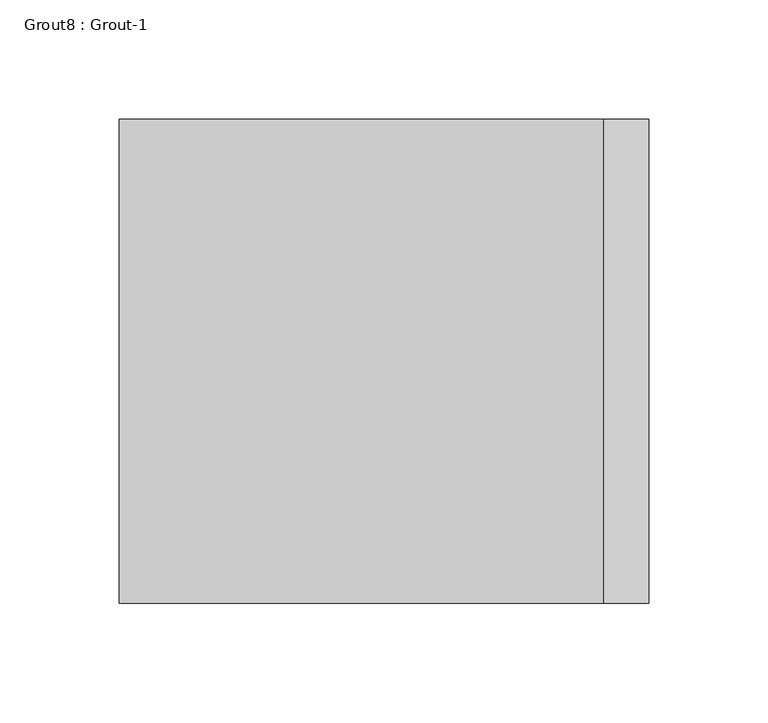
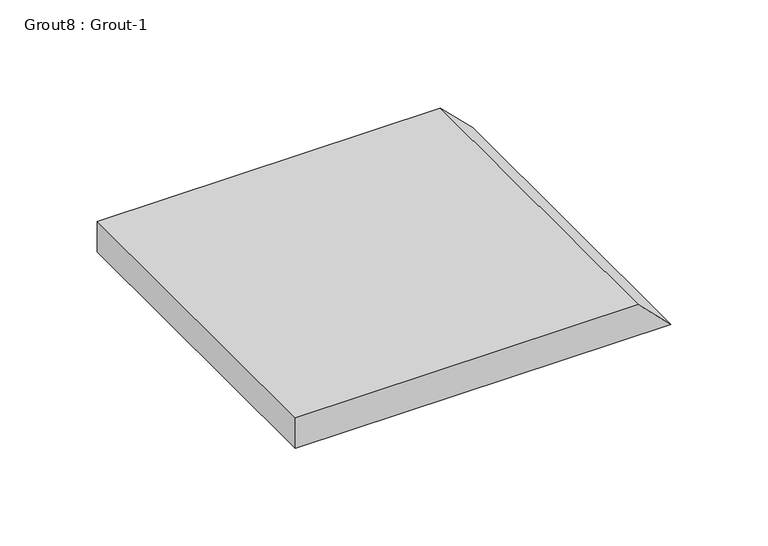
"""IFC4 building model written with IfcOpenShell, lengths in millimetres: proxy geometry, Grout8 : Grout-1."""

import ifcopenshell
import ifcopenshell.guid

model = None  # the IFC model being written
_history = None  # IfcOwnerHistory: only IFC2X3 demands one
_inside = {}  # id of a spatial element -> (the spatial element, [elements in it])
_under = {}  # id of a project, library or spatial element -> (it, [spatial elements below it])
_declared = {}  # id of a project -> (the project, [libraries it declares])
_typed = {}  # id of a type object -> (the type object, [elements of that type])
_made_of = {}  # id of a material, layer set ... -> (it, [elements and type objects made of it])


def new_model(schema):
    """Start an empty IFC model of exactly this schema.

    Asked for "IFC4X3", IfcOpenShell would pick the latest addendum, in which some entities
    have other attributes; the version numbers below select the first issue.
    IFC2X3 requires an IfcOwnerHistory on every rooted entity: one is made here for all.
    """
    global model, _history
    if schema == "IFC4X3":
        model = ifcopenshell.file(schema_version=(4, 3, 0, 0))
    else:
        model = ifcopenshell.file(schema=schema)
    _inside.clear()
    _under.clear()
    _declared.clear()
    _typed.clear()
    _made_of.clear()
    _history = None
    if model.schema == "IFC2X3":
        org = make("IfcOrganization", Name="unknown")
        user = make(
            "IfcPersonAndOrganization",
            ThePerson=make("IfcPerson", FamilyName="unknown"),
            TheOrganization=org,
        )
        app = make(
            "IfcApplication",
            ApplicationDeveloper=org,
            Version="unknown",
            ApplicationFullName="unknown",
            ApplicationIdentifier="unknown",
        )
        _history = make(
            "IfcOwnerHistory",
            OwningUser=user,
            OwningApplication=app,
            ChangeAction="ADDED",
            CreationDate=0,
        )
    return model


def make(cls, **values):
    """One entity of the class cls with the attributes given. An attribute that is None is left unset."""
    return model.create_entity(
        cls, **{name: value for name, value in values.items() if value is not None}
    )


def rooted(cls, **values):
    """An entity with a GlobalId (a new one), such as an element, a storey or a relation."""
    return make(cls, GlobalId=ifcopenshell.guid.new(), OwnerHistory=_history, **values)


def si_unit(unit_type, name, prefix=None):
    """IfcSIUnit, for example si_unit("LENGTHUNIT", "METRE", prefix="MILLI")."""
    return make("IfcSIUnit", UnitType=unit_type, Prefix=prefix, Name=name)


def assignment(units):
    """IfcUnitAssignment: the units of a project."""
    return None if units is None else make("IfcUnitAssignment", Units=units)


def point(xyz):
    """IfcCartesianPoint."""
    return None if xyz is None else make("IfcCartesianPoint", Coordinates=xyz)


def direction(xyz):
    """IfcDirection."""
    return None if xyz is None else make("IfcDirection", DirectionRatios=xyz)


def frame(location, z_axis=None, x_axis=None):
    """IfcAxis2Placement3D, a coordinate frame: its origin and axes. An axis left out is left unset."""
    return make(
        "IfcAxis2Placement3D",
        Location=point(location),
        Axis=direction(z_axis),
        RefDirection=direction(x_axis),
    )


def origin():
    """The frame at (0, 0, 0) with its axes left unset."""
    return frame((0.0, 0.0, 0.0))


def place(relative_to, where):
    """IfcLocalPlacement: puts the frame where relative to a parent placement (None: the world)."""
    return make(
        "IfcLocalPlacement", PlacementRelTo=relative_to, RelativePlacement=where
    )


def context(
    kind, dimensions, precision=None, world=None, true_north=None, identifier=None
):
    """IfcGeometricRepresentationContext, for example the 3D "Model" context."""
    return make(
        "IfcGeometricRepresentationContext",
        ContextIdentifier=identifier,
        ContextType=kind,
        CoordinateSpaceDimension=dimensions,
        Precision=precision,
        WorldCoordinateSystem=world,
        TrueNorth=true_north,
    )


def project(units=None, contexts=None):
    """IfcProject with its units and contexts."""
    return rooted(
        "IfcProject",
        Name="project",
        RepresentationContexts=contexts,
        UnitsInContext=assignment(units),
    )


def spatial(cls, under=None, at=None, **own):
    """A site, building, storey or space (cls), placed at a placement, below another one or the project."""
    s = rooted(cls, ObjectPlacement=at, **own)
    if under is not None:
        _under.setdefault(under.id(), (under, []))[1].append(s)
    return s


def polyline(points):
    """IfcPolyline through the points."""
    return make("IfcPolyline", Points=[point(p) for p in points])


def outline(outer, holes=None, kind="AREA"):
    """IfcArbitraryClosedProfileDef: a profile drawn as a closed curve; with holes, ...WithVoids."""
    if holes is None:
        return make("IfcArbitraryClosedProfileDef", ProfileType=kind, OuterCurve=outer)
    return make(
        "IfcArbitraryProfileDefWithVoids",
        ProfileType=kind,
        OuterCurve=outer,
        InnerCurves=holes,
    )


def extrude(swept, where, along, depth):
    """IfcExtrudedAreaSolid: the profile swept, set in the frame where, extruded along a direction by depth."""
    return make(
        "IfcExtrudedAreaSolid",
        SweptArea=swept,
        Position=where,
        ExtrudedDirection=direction(along),
        Depth=depth,
    )


def shape(context_of_items, identifier, shape_type, items):
    """IfcShapeRepresentation: the items that make up one representation, for example the "Body"."""
    return make(
        "IfcShapeRepresentation",
        ContextOfItems=context_of_items,
        RepresentationIdentifier=identifier,
        RepresentationType=shape_type,
        Items=items,
    )


def source(mapping_origin, context_of_items, identifier, shape_type, items):
    """IfcRepresentationMap: a shape defined once, which mapped items show again and again."""
    return make(
        "IfcRepresentationMap",
        MappingOrigin=mapping_origin,
        MappedRepresentation=shape(context_of_items, identifier, shape_type, items),
    )


def transform(
    local_origin,
    x_axis=None,
    y_axis=None,
    z_axis=None,
    scale=None,
    scale2=None,
    scale3=None,
    uniform=True,
):
    """IfcCartesianTransformationOperator3D, or its non-uniform kind. x_axis, y_axis, z_axis: its Axis1, 2, 3."""
    if uniform:
        return make(
            "IfcCartesianTransformationOperator3D",
            Axis1=direction(x_axis),
            Axis2=direction(y_axis),
            LocalOrigin=point(local_origin),
            Scale=scale,
            Axis3=direction(z_axis),
        )
    return make(
        "IfcCartesianTransformationOperator3DnonUniform",
        Axis1=direction(x_axis),
        Axis2=direction(y_axis),
        LocalOrigin=point(local_origin),
        Scale=scale,
        Axis3=direction(z_axis),
        Scale2=scale2,
        Scale3=scale3,
    )


def mapped(mapping_source, mapping_target):
    """IfcMappedItem: shows the shape of a source again, moved by a transform."""
    return make(
        "IfcMappedItem", MappingSource=mapping_source, MappingTarget=mapping_target
    )


def made_of(thing, what):
    """Note that an element or type object is made of a material, layer set ...; save() writes the relation."""
    if what is not None:
        _made_of.setdefault(what.id(), (what, []))[1].append(thing)
    return thing


def element(
    cls,
    number,
    at=None,
    inside=None,
    cuts=None,
    type_object=None,
    material=None,
    context=None,
    identifier="Body",
    shape_type=None,
    held_by="IfcProductDefinitionShape",
    body=None,
    shapes=None,
    **own,
):
    """One element of the class cls, such as IfcWall. Its Tag is "e" and its number.

    at: its placement. inside: the storey or other place that contains it. cuts: it is an
    opening in that element (IfcRelVoidsElement). A single representation is given by context,
    identifier, shape_type and body (its items); several are given by shapes. held_by: the class
    of the entity that holds the representations. save() writes the other relations.
    """
    e = rooted(cls, Tag="e%d" % number, ObjectPlacement=at, **own)
    if body is not None:
        shapes = [shape(context, identifier, shape_type, body)]
    if shapes is not None:
        e.Representation = make(held_by, Representations=shapes)
    if inside is not None:
        _inside.setdefault(inside.id(), (inside, []))[1].append(e)
    if cuts is not None:
        rooted(
            "IfcRelVoidsElement", RelatingBuildingElement=cuts, RelatedOpeningElement=e
        )
    if type_object is not None:
        _typed.setdefault(type_object.id(), (type_object, []))[1].append(e)
    return made_of(e, material)


def aggregate(whole, parts):
    """IfcRelAggregates: a whole, such as a stair, and the parts it consists of."""
    return rooted("IfcRelAggregates", RelatingObject=whole, RelatedObjects=parts)


def save(model, path):
    """Write the relations noted so far, then the file.

    IfcRelAggregates (storeys below a building ...), IfcRelContainedInSpatialStructure (elements
    in a storey), IfcRelDefinesByType, IfcRelAssociatesMaterial and IfcRelDeclares: one each for
    every whole, place, type object, material and project.
    """
    for whole, parts in _under.values():
        aggregate(whole, parts)
    for where, things in _inside.values():
        rooted(
            "IfcRelContainedInSpatialStructure",
            RelatedElements=things,
            RelatingStructure=where,
        )
    for kind, things in _typed.values():
        rooted("IfcRelDefinesByType", RelatedObjects=things, RelatingType=kind)
    for what, things in _made_of.values():
        rooted("IfcRelAssociatesMaterial", RelatedObjects=things, RelatingMaterial=what)
    for by, libraries in _declared.values():
        rooted("IfcRelDeclares", RelatingContext=by, RelatedDefinitions=libraries)
    model.write(path)


def grout8_grout_1_13d29c56(model_context):
    return source(origin(), model_context, "Body", "SweptSolid", [
        extrude(outline(polyline([(19.05, 587569.0934739), (19.05, 587365.8934739), (0.0, 587365.8934739), (0.0, 587588.1434739), (19.05, 587569.0934739)])), frame((0.0, -536468.3913841, 0.0), z_axis=(0.0, 1.0, 0.0), x_axis=(0.0, 0.0, 1.0)), (0.0, 0.0, 1.0), 203.2),
    ])


if __name__ == "__main__":
    model = new_model("IFC4")
    model_context = context("Model", 3, world=origin())
    ifc_project = project(units=[si_unit("LENGTHUNIT", "METRE", prefix="MILLI")], contexts=[model_context])
    site = spatial("IfcSite", under=ifc_project)
    building = spatial("IfcBuilding", under=site)
    placement = place(None, origin())
    grout8_grout_1_shape = grout8_grout_1_13d29c56(model_context)
    element("IfcBuildingElementProxy", 1, Name="Grout8 : Grout-1", ObjectType="Grout8 : Grout-1", at=placement, inside=building, context=model_context, shape_type="MappedRepresentation", body=[
        mapped(grout8_grout_1_shape, transform((0.0, 0.0, 0.0), x_axis=(1.0, 0.0, 0.0), y_axis=(0.0, 1.0, 0.0), z_axis=(0.0, 0.0, 1.0))),
    ])
    save(model, "model.ifc")

# Revit data of these elements
# Element 1 (IfcBuildingElementProxy, "Grout8 : Grout-1")
#   Materials on its faces: "3/4\" NON SHRINK GROUT"
# Materials
#   "3/4\" NON SHRINK GROUT": class "Generic", colour RGB 145 145 143, transparency 0, Cost = 0
